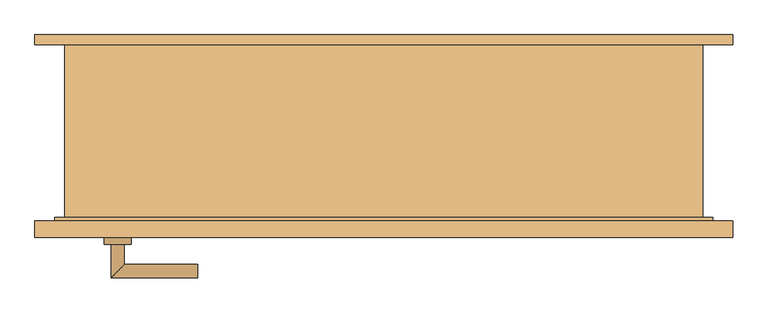
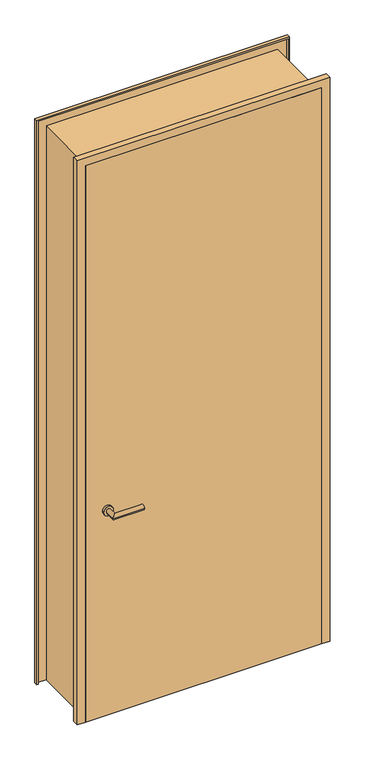
"""IFC4 building model written with IfcOpenShell, lengths in millimetres: door geometry, Drehflügel 1-flg - Stahlzarge : Holztüre 1,0 x 2,45."""

from ifc_helpers import new_model, si_unit, point, frame, frame_2d, origin, place, context, project, spatial, polyline, circle_curve, ellipse_curve, trimmed, segment, composite_curve, outline, extrude, faceted_brep, source, transform, mapped, element, save
from ifc_brep_helpers import plane_surface, cylinder_surface, advanced_brep


def door_a1bbb9cb(model_context):
    return source(origin(), model_context, "Body", "SolidModel", [
        advanced_brep(
        [(-410.0, -121.9346141, 1000.0), (-390.0, -121.9346141, 1000.0), (-390.0, -71.9346141, 1000.0), (-410.0, -51.9346141, 1000.0), (-280.0, -51.9346141, 1000.0), (-280.0, -71.9346141, 1000.0)],
        [
            (0, 1, circle_curve(frame((-400.0, -121.9346141, 1000.0), z_axis=(0.0, -1.0, 0.0), x_axis=(1.0, 0.0, 0.0)), 10.0)),
            (1, 0, circle_curve(frame((-400.0, -121.9346141, 1000.0), z_axis=(0.0, -1.0, 0.0), x_axis=(1.0, 0.0, 0.0)), 10.0)),
            (1, 2),
            (2, 3, ellipse_curve(frame((-400.0, -61.9346141, 1000.0), z_axis=(-0.7071067811865385, -0.7071067811865565, 0.0), x_axis=(0.7071067811865563, -0.7071067811865386, 0.0)), 14.1421356, 10.0)),
            (3, 0),
            (3, 2, ellipse_curve(frame((-400.0, -61.9346141, 1000.0), z_axis=(-0.7071067811865385, -0.7071067811865565, 0.0), x_axis=(0.7071067811865563, -0.7071067811865386, 0.0)), 14.1421356, 10.0)),
            (4, 5, circle_curve(frame((-280.0, -61.9346141, 1000.0), z_axis=(1.0, 0.0, 0.0), x_axis=(0.0, -1.0, 0.0)), 10.0)),
            (5, 4, circle_curve(frame((-280.0, -61.9346141, 1000.0), z_axis=(1.0, 0.0, 0.0), x_axis=(0.0, -1.0, 0.0)), 10.0)),
            (2, 5),
            (4, 3),
        ],
        [
            plane_surface(frame((-400.0, -121.9346141, -287.7526403), z_axis=(0.0, -1.0, 0.0), x_axis=(0.0, 0.0, 1.0))),
            cylinder_surface(frame((-400.0, -121.9346141, 1000.0), z_axis=(0.0, -1.0, 0.0), x_axis=(1.0, 0.0, 0.0)), 10.0),
            plane_surface(frame((-280.0, -61.9346141, -287.7526403), z_axis=(1.0, 0.0, 0.0), x_axis=(0.0, 0.0, 1.0))),
            cylinder_surface(frame((-400.0, -61.9346141, 1000.0), z_axis=(-1.0, 0.0, 0.0), x_axis=(0.0, -1.0, 0.0)), 10.0),
        ],
        [
            (0, [[1, 2]]),
            (1, [[3, 4, 5, -2]]),
            (1, [[-5, 6, -3, -1]]),
            (2, [[7, 8]]),
            (3, [[9, -7, 10, -4]]),
            (3, [[-10, -8, -9, -6]]),
        ],
    ),
        advanced_brep(
        [(-390.0, -181.9346141, 1000.0), (-410.0, -181.9346141, 1000.0), (-410.0, -231.9346141, 1000.0), (-390.0, -211.9346141, 1000.0), (-280.0, -211.9346141, 1000.0), (-280.0, -231.9346141, 1000.0)],
        [
            (0, 1, circle_curve(frame((-400.0, -181.9346141, 1000.0), z_axis=(0.0, 1.0, 0.0), x_axis=(-1.0, 0.0, 0.0)), 10.0)),
            (1, 0, circle_curve(frame((-400.0, -181.9346141, 1000.0), z_axis=(0.0, 1.0, 0.0), x_axis=(-1.0, 0.0, 0.0)), 10.0)),
            (1, 2),
            (2, 3, ellipse_curve(frame((-400.0, -221.9346141, 1000.0), z_axis=(-0.7071067811865475, 0.7071067811865475, 0.0), x_axis=(0.7071067811865474, 0.7071067811865476, 0.0)), 14.1421356, 10.0)),
            (3, 0),
            (3, 2, ellipse_curve(frame((-400.0, -221.9346141, 1000.0), z_axis=(-0.7071067811865475, 0.7071067811865475, 0.0), x_axis=(0.7071067811865474, 0.7071067811865476, 0.0)), 14.1421356, 10.0)),
            (4, 5, circle_curve(frame((-280.0, -221.9346141, 1000.0), z_axis=(1.0, 0.0, 0.0), x_axis=(0.0, -1.0, 0.0)), 10.0)),
            (5, 4, circle_curve(frame((-280.0, -221.9346141, 1000.0), z_axis=(1.0, 0.0, 0.0), x_axis=(0.0, -1.0, 0.0)), 10.0)),
            (2, 5),
            (4, 3),
        ],
        [
            plane_surface(frame((-400.0, -181.9346141, -287.7526403), z_axis=(0.0, 1.0, 0.0), x_axis=(0.0, 0.0, 1.0))),
            cylinder_surface(frame((-400.0, -181.9346141, 1000.0), z_axis=(0.0, 1.0, 0.0), x_axis=(-1.0, 0.0, 0.0)), 10.0),
            plane_surface(frame((-280.0, -221.9346141, -287.7526403), z_axis=(1.0, 0.0, 0.0), x_axis=(0.0, 0.0, 1.0))),
            cylinder_surface(frame((-400.0, -221.9346141, 1000.0), z_axis=(-1.0, 0.0, 0.0), x_axis=(0.0, -1.0, 0.0)), 10.0),
        ],
        [
            (0, [[1, 2]]),
            (1, [[3, 4, 5, -2]]),
            (1, [[-5, 6, -3, -1]]),
            (2, [[7, 8]]),
            (3, [[9, -7, 10, -4]]),
            (3, [[-10, -8, -9, -6]]),
        ],
    ),
        extrude(outline(composite_curve([segment(trimmed(circle_curve(frame_2d((1000.0, -400.0)), 20.0), [point((1000.0, -420.0))], [point((1000.0, -380.0))], False, "CARTESIAN"), True, "CONTINUOUS"), segment(trimmed(circle_curve(frame_2d((1000.0, -400.0)), 20.0), [point((1000.0, -380.0))], [point((1000.0, -420.0))], False, "CARTESIAN"), True, "CONTINUOUS")], self_intersect=False)), frame((0.0, -121.9346141, 0.0), z_axis=(0.0, 1.0, 0.0), x_axis=(0.0, 0.0, 1.0)), (0.0, 0.0, 1.0), 10.0),
        extrude(outline(composite_curve([segment(trimmed(circle_curve(frame_2d((1000.0, -400.0)), 20.0), [point((1000.0, -420.0))], [point((1000.0, -380.0))], False, "CARTESIAN"), True, "CONTINUOUS"), segment(trimmed(circle_curve(frame_2d((1000.0, -400.0)), 20.0), [point((1000.0, -380.0))], [point((1000.0, -420.0))], False, "CARTESIAN"), True, "CONTINUOUS")], self_intersect=False)), frame((0.0, -181.9346141, 0.0), z_axis=(0.0, 1.0, 0.0), x_axis=(0.0, 0.0, 1.0)), (0.0, 0.0, 1.0), 10.0),
        extrude(outline(polyline([(490.0, -146.9346141), (490.0, -171.9346141), (-490.0, -171.9346141), (-490.0, -146.9346141), (490.0, -146.9346141)])), frame((0.0, 0.0, 100.0), z_axis=(0.0, 0.0, 1.0), x_axis=(1.0, 0.0, 0.0)), (0.0, 0.0, 1.0), 2440.0),
        faceted_brep([(524.4603207, 133.0653859, 100.0), (524.4603207, 118.0653859, 100.0), (519.4603207, 118.0653859, 100.0), (519.4603207, 128.0653859, 100.0), (480.0, 128.0653859, 100.0), (480.0, -141.9346141, 100.0), (495.0, -141.9346141, 100.0), (495.0, -166.9346141, 100.0), (519.4603207, -166.9346141, 100.0), (519.4603207, -146.9346141, 100.0), (524.4603207, -146.9346141, 100.0), (524.4603207, -171.9346141, 100.0), (490.0, -171.9346141, 100.0), (490.0, -146.9346141, 100.0), (475.0, -146.9346141, 100.0), (475.0, 133.0653859, 100.0), (475.0, 133.0653859, 2525.0), (-475.0, 133.0653859, 2525.0), (-475.0, 133.0653859, 100.0), (-524.4603207, 133.0653859, 100.0), (-524.4603207, 133.0653859, 2574.4603207), (524.4603207, 133.0653859, 2574.4603207), (475.0, -146.9346141, 2525.0), (490.0, -146.9346141, 2540.0), (-490.0, -146.9346141, 2540.0), (-490.0, -146.9346141, 100.0), (-475.0, -146.9346141, 100.0), (-475.0, -146.9346141, 2525.0), (490.0, -171.9346141, 2540.0), (524.4603207, -171.9346141, 2574.4603207), (-524.4603207, -171.9346141, 2574.4603207), (-524.4603207, -171.9346141, 100.0), (-490.0, -171.9346141, 100.0), (-490.0, -171.9346141, 2540.0), (524.4603207, -146.9346141, 2574.4603207), (519.4603207, -146.9346141, 2569.4603207), (-519.4603207, -146.9346141, 2569.4603207), (-519.4603207, -146.9346141, 100.0), (-524.4603207, -146.9346141, 100.0), (-524.4603207, -146.9346141, 2574.4603207), (519.4603207, -166.9346141, 2569.4603207), (495.0, -166.9346141, 2545.0), (-495.0, -166.9346141, 2545.0), (-495.0, -166.9346141, 100.0), (-519.4603207, -166.9346141, 100.0), (-519.4603207, -166.9346141, 2569.4603207), (495.0, -141.9346141, 2545.0), (480.0, -141.9346141, 2530.0), (-480.0, -141.9346141, 2530.0), (-480.0, -141.9346141, 100.0), (-495.0, -141.9346141, 100.0), (-495.0, -141.9346141, 2545.0), (480.0, 128.0653859, 2530.0), (519.4603207, 128.0653859, 2569.4603207), (-519.4603207, 128.0653859, 2569.4603207), (-519.4603207, 128.0653859, 100.0), (-480.0, 128.0653859, 100.0), (-480.0, 128.0653859, 2530.0), (519.4603207, 118.0653859, 2569.4603207), (524.4603207, 118.0653859, 2574.4603207), (-524.4603207, 118.0653859, 2574.4603207), (-524.4603207, 118.0653859, 100.0), (-519.4603207, 118.0653859, 100.0), (-519.4603207, 118.0653859, 2569.4603207)], [[[0, 1, 2, 3, 4, 5, 6, 7, 8, 9, 10, 11, 12, 13, 14, 15]], [[15, 16, 17, 18, 19, 20, 21, 0]], [[14, 22, 16, 15]], [[13, 23, 24, 25, 26, 27, 22, 14]], [[12, 28, 23, 13]], [[11, 29, 30, 31, 32, 33, 28, 12]], [[10, 34, 29, 11]], [[9, 35, 36, 37, 38, 39, 34, 10]], [[8, 40, 35, 9]], [[7, 41, 42, 43, 44, 45, 40, 8]], [[6, 46, 41, 7]], [[5, 47, 48, 49, 50, 51, 46, 6]], [[4, 52, 47, 5]], [[3, 53, 54, 55, 56, 57, 52, 4]], [[2, 58, 53, 3]], [[1, 59, 60, 61, 62, 63, 58, 2]], [[0, 21, 59, 1]], [[20, 19, 61, 60]], [[19, 18, 26, 25, 32, 31, 38, 37, 44, 43, 50, 49, 56, 55, 62, 61]], [[27, 26, 18, 17]], [[33, 32, 25, 24]], [[39, 38, 31, 30]], [[45, 44, 37, 36]], [[51, 50, 43, 42]], [[57, 56, 49, 48]], [[63, 62, 55, 54]], [[22, 27, 17, 16]], [[28, 33, 24, 23]], [[34, 39, 30, 29]], [[40, 45, 36, 35]], [[46, 51, 42, 41]], [[52, 57, 48, 47]], [[58, 63, 54, 53]], [[21, 20, 60, 59]]]),
    ])


if __name__ == "__main__":
    model = new_model("IFC4")
    model_context = context("Model", 3, world=origin())
    ifc_project = project(units=[si_unit("LENGTHUNIT", "METRE", prefix="MILLI")], contexts=[model_context])
    site = spatial("IfcSite", under=ifc_project)
    building = spatial("IfcBuilding", under=site)
    placement = place(None, origin())
    door_shape = door_a1bbb9cb(model_context)
    element("IfcDoor", 1, ObjectType="Drehflügel 1-flg - Stahlzarge : Holztüre 1,0 x 2,45", at=placement, inside=building, context=model_context, shape_type="MappedRepresentation", body=[
        mapped(door_shape, transform((0.0, 0.0, 0.0), x_axis=(1.0, 0.0, 0.0), y_axis=(0.0, 1.0, 0.0), z_axis=(0.0, 0.0, 1.0))),
    ])
    save(model, "model.ifc")

# Revit data of these elements
# Type "Drehflügel 1-flg - Stahlzarge : Holztüre 1,0 x 2,45"
#   Type Mark = "23"
#   Operation = "SingleSwingRight"
#   Keynote = "16.03"
#   Analytic Construction = "Metall"
#   Thermal Resistance (R) = 0.270117 (m²·K)/W
#   Heat Transfer Coefficient (U) = 3.7021 W/(m²·K)
#   Rough Width = 1.000 m
#   Rough Height [instance default] = 2.550 m
#   Höhe Türgriff [instance default] = 0.900 m
#   Height = 2.450 m
#   Fußbodenaufbau [instance default] = 0.100 m
#   Width = 1.000 m
#   Sichtbarkeit Sturzlinien [instance default] = yes
#   Türgriff auswählen [instance default] = element 221079
#   Türgriff [instance default] = none
#   Türflügel [instance default] = none
#   Rahmen/Pfosten [instance default] = Metall - Lackiert - Grau
#   Visual Light Transmittance = 0
#   Solar Heat Gain Coefficient = 0
#   Function = (empty or 0)
#   Wall Closure = (empty or 0)
# Element 1 (IfcDoor, "Drehflügel 1-flg - Stahlzarge : Holztüre 1,0 x 2,45")
#   Materials on its faces: "Metall - Lackiert - Grau", "Metall - Chrom", "Holz - Birke"
# Materials
#   "Metall - Lackiert - Grau": class "Farbe 1", colour RGB 98 98 98, transparency 0, Cost = 0
#   "Metall - Chrom": class "Metall", colour RGB 247 247 247, transparency 0, Cost = 0
#   "Holz - Birke": class "Holz", colour RGB 213 164 103, transparency 0, Cost = 0
